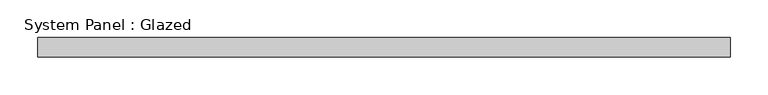
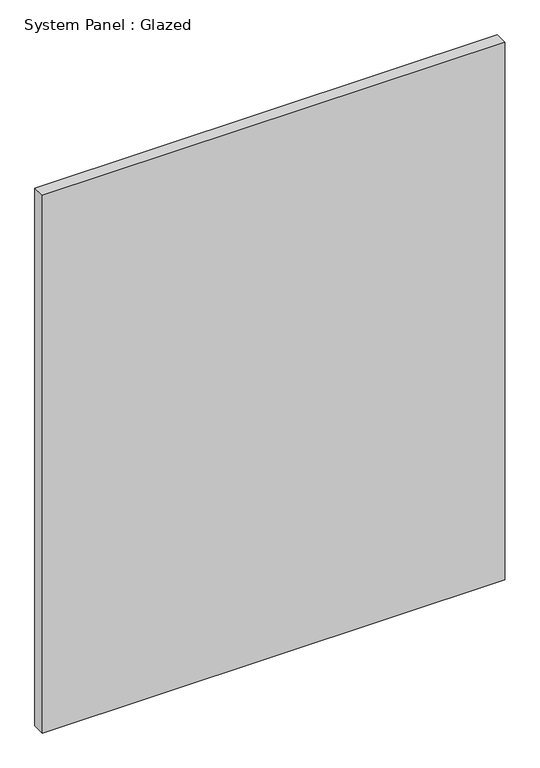
"""IFC4 building model written with IfcOpenShell, lengths in millimetres: plate geometry, System Panel : Glazed."""

from ifc_helpers import new_model, si_unit, origin, origin_with_axes, place, context, project, spatial, polyline, outline, extrude, source, transform, mapped, element, save


def system_panel_glazed_1925881f(model_context):
    return source(origin(), model_context, "Body", "SweptSolid", [
        extrude(outline(polyline([(457.2, 19.05), (-457.2, 19.05), (-457.2, 44.45), (457.2, 44.45), (457.2, 19.05)])), origin_with_axes(), (0.0, 0.0, 1.0), 1123.95),
    ])


if __name__ == "__main__":
    model = new_model("IFC4")
    model_context = context("Model", 3, world=origin())
    ifc_project = project(units=[si_unit("LENGTHUNIT", "METRE", prefix="MILLI")], contexts=[model_context])
    site = spatial("IfcSite", under=ifc_project)
    building = spatial("IfcBuilding", under=site)
    placement = place(None, origin())
    system_panel_glazed_shape = system_panel_glazed_1925881f(model_context)
    element("IfcPlate", 1, ObjectType="System Panel : Glazed", at=placement, inside=building, context=model_context, shape_type="MappedRepresentation", body=[
        mapped(system_panel_glazed_shape, transform((0.0, 0.0, 0.0), x_axis=(1.0, 0.0, 0.0), y_axis=(0.0, 1.0, 0.0), z_axis=(0.0, 0.0, 1.0))),
    ])
    save(model, "model.ifc")

# Revit data of these elements
# Element 1 (IfcPlate, "System Panel : Glazed")
#   Materials on its faces: "Glass"
# Materials
#   "Glass": class "Glass", colour RGB 0 128 192, transparency 0.75
